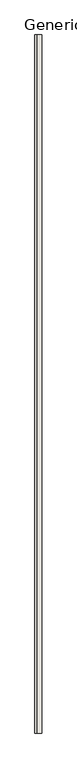
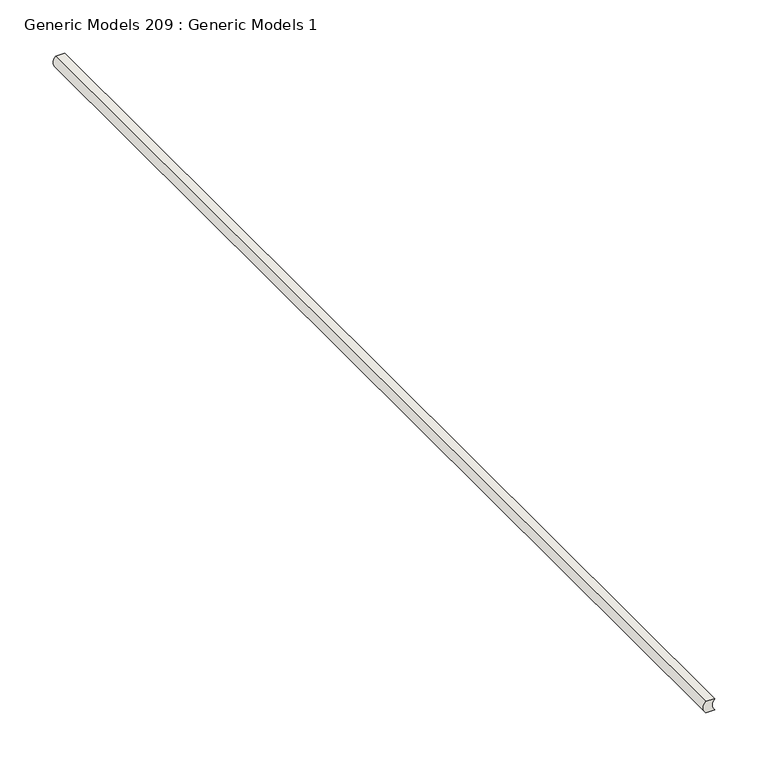
"""IFC4 building model written with IfcOpenShell, lengths in millimetres: wall geometry, Generic Models 209 : Generic Models 1."""

from ifc_helpers import new_model, si_unit, point, frame, frame_2d, origin, place, context, project, spatial, polyline, circle_curve, trimmed, segment, composite_curve, outline, extrude, source, transform, mapped, element, save


def generic_models_209_generic_models_1_1f6e0a5c(model_context):
    return source(origin(), model_context, "Body", "SweptSolid", [
        extrude(outline(composite_curve([segment(trimmed(circle_curve(frame_2d((2451.1, 141245.704481)), 8.620055), [point((2444.75, 141239.875))], [point((2457.45, 141239.875))], True, "CARTESIAN"), True, "CONTINUOUS"), segment(polyline([(2457.45, 141239.875), (2457.45, 141230.35)]), True, "CONTINUOUS"), segment(trimmed(circle_curve(frame_2d((2451.1, 141236.179481)), 8.620055), [point((2457.45, 141230.35))], [point((2444.75, 141230.35))], False, "CARTESIAN"), True, "CONTINUOUS"), segment(polyline([(2444.75, 141230.35), (2444.75, 141239.875)]), True, "CONTINUOUS")], self_intersect=False)), frame((0.0, 0.0, 0.0), z_axis=(0.0, 1.0, 0.0), x_axis=(0.0, 0.0, 1.0)), (0.0, 0.0, 1.0), 1219.2),
    ])


if __name__ == "__main__":
    model = new_model("IFC4")
    model_context = context("Model", 3, world=origin())
    ifc_project = project(units=[si_unit("LENGTHUNIT", "METRE", prefix="MILLI")], contexts=[model_context])
    site = spatial("IfcSite", under=ifc_project)
    building = spatial("IfcBuilding", under=site)
    placement = place(None, origin())
    generic_models_209_generic_models_1_shape = generic_models_209_generic_models_1_1f6e0a5c(model_context)
    element("IfcWall", 1, ObjectType="Generic Models 209 : Generic Models 1", at=placement, inside=building, context=model_context, shape_type="MappedRepresentation", body=[
        mapped(generic_models_209_generic_models_1_shape, transform((0.0, 0.0, 0.0), x_axis=(1.0, 0.0, 0.0), y_axis=(0.0, 1.0, 0.0), z_axis=(0.0, 0.0, 1.0))),
    ])
    save(model, "model.ifc")

# Revit data of these elements
# Element 1 (IfcWall, "Generic Models 209 : Generic Models 1")
#   Materials on its faces: "ACOUSTICAL SEALANT OR FIRE SEALANT, IF RATED WALL"
# Materials
#   "ACOUSTICAL SEALANT OR FIRE SEALANT, IF RATED WALL": class "Unassigned", colour RGB 120 120 120, transparency 0, Cost = 0
